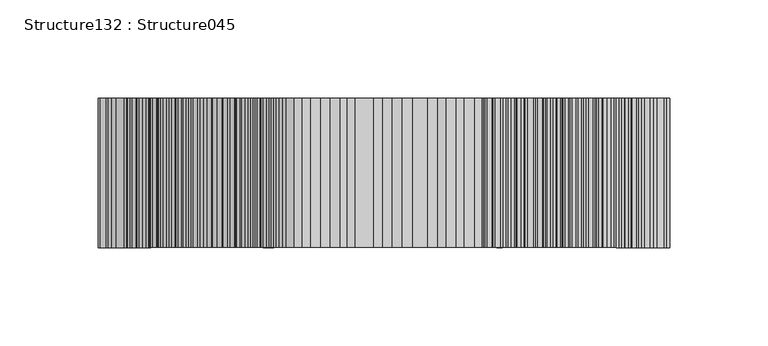
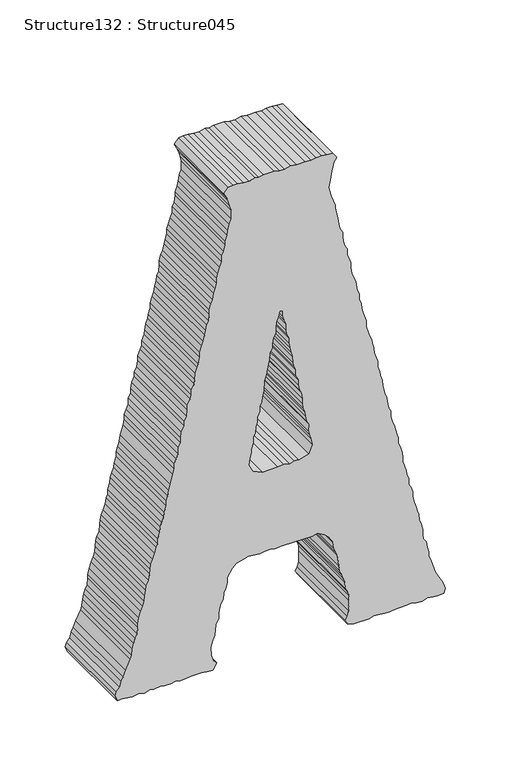
"""IFC4 building model written with IfcOpenShell, lengths in millimetres: proxy geometry, Structure132 : Structure045."""

from ifc_helpers import new_model, si_unit, frame, origin, place, context, project, spatial, polyline, outline, extrude, source, transform, mapped, element, save


def structure132_structure045_523e0b6c(model_context):
    return source(origin(), model_context, "Body", "SweptSolid", [
        extrude(outline(polyline([(3818.8310229, -44517.1979045), (3814.7296538, -44517.1979045), (3811.2043377, -44518.372475), (3805.9476534, -44520.7151975), (3801.8462843, -44520.7151975), (3795.960595, -44521.297669), (3791.8865042, -44523.6387869), (3787.7867397, -44523.6387869), (3783.0868532, -44525.9911371), (3777.8285642, -44526.5655855), (3773.11905, -44526.5655855), (3769.6274306, -44528.9147265), (3763.759392, -44528.9147265), (3759.6596275, -44530.6637454), (3755.559863, -44532.430415), (3750.8583719, -44532.430415), (3746.1745313, -44533.598567), (3737.400554, -44535.9509172), (3732.1149867, -44537.1158601), (3727.4311462, -44538.280803), (3723.3313817, -44539.4585827), (3718.6571688, -44539.4585827), (3713.3555556, -44541.2156246), (3709.2718371, -44541.7997006), (3704.5879966, -44543.5679748), (3701.0723082, -44544.7248946), (3695.786741, -44545.3169937), (3690.512406, -44547.0756402), (3685.8285655, -44547.0756402), (3682.8857208, -44548.2502107), (3677.6274319, -44549.4183628), (3672.9435914, -44551.1850323), (3668.8261762, -44552.9340512), (3664.1423357, -44553.5165226), (3660.0682449, -44554.1086217), (3654.1841602, -44554.6926977), (3650.1004418, -44557.0354203), (3645.9830266, -44557.6162871), (3641.2991861, -44558.2099908), (3636.0408972, -44558.8004853), (3631.915459, -44559.9590097), (3627.8397636, -44561.7256792), (3622.555801, -44563.4843258), (3617.2718384, -44564.6508732), (3613.772196, -44564.6508732), (3607.8961343, -44565.2349493), (3604.3964919, -44567.0016188), (3600.2967274, -44568.1697709), (3595.5872132, -44569.3443414), (3589.7544759, -44569.9284174), (3586.2115092, -44571.0933603), (3577.4535778, -44575.1931248), (3572.1423369, -44577.545475), (3568.6426945, -44579.3041215), (3563.366755, -44580.4690644), (3560.441561, -44583.403886), (3556.3417965, -44584.5784565), (3551.6675836, -44582.8117869), (3551.6675836, -44578.1359694), (3551.0658569, -44573.4441059), (3550.4833855, -44569.3443414), (3551.6675836, -44564.0684018), (3550.4833855, -44558.8004853), (3551.6675836, -44554.1086217), (3551.0658569, -44550.5929333), (3551.6675836, -44544.7248946), (3551.0658569, -44541.2156246), (3551.0658569, -44535.3572136), (3551.6675836, -44531.2574491), (3551.0658569, -44527.1464524), (3551.0658569, -44522.4642164), (3551.6675836, -44517.7803759), (3551.6675836, -44508.4046719), (3551.0658569, -44503.7128083), (3550.4833855, -44498.4448918), (3556.3417965, -44494.9275987), (3559.2669905, -44497.8624203), (3565.1254015, -44499.6210668), (3572.7440636, -44500.1971199), (3578.6104977, -44498.4448918), (3582.7102621, -44496.6782222), (3587.3860796, -44496.0957508), (3592.0955938, -44495.5213024), (3596.7698067, -44493.1689522), (3601.4536473, -44493.1689522), (3604.9709403, -44492.5784577), (3610.2292293, -44491.4119102), (3613.772196, -44489.0627693), (3619.6145609, -44488.4867163), (3622.555801, -44486.7296743), (3627.8397636, -44485.5518946), (3633.0980525, -44485.5518946), (3639.5405396, -44480.8696587), (3643.0578326, -44477.3443426), (3644.8245022, -44470.3177795), (3645.9830266, -44466.8004865), (3645.4262289, -44460.9420755), (3644.8245022, -44456.8407064), (3645.4262289, -44452.1504474), (3645.9830266, -44447.4650023), (3644.8245022, -44443.3748655), (3645.4262289, -44438.0892983), (3645.4262289, -44425.7900048), (3644.8245022, -44419.9299892), (3644.8245022, -44410.5542851), (3645.9830266, -44405.8704446), (3642.4833842, -44399.4199345), (3638.9580681, -44395.32017), (3633.0980525, -44392.3965806), (3627.2396415, -44391.2107779), (3622.555801, -44389.4601544), (3619.6145609, -44388.2871885), (3609.0723094, -44387.1190364), (3604.3964919, -44385.952489), (3600.2967274, -44384.7779185), (3596.1953583, -44383.0176674), (3592.0955938, -44381.8430969), (3586.2115092, -44381.2590208), (3582.7102621, -44379.5019789), (3578.6104977, -44378.3274084), (3573.9266571, -44378.3274084), (3563.9412034, -44378.3274084), (3559.2669905, -44379.5019789), (3555.7416744, -44381.2590208), (3551.6675836, -44378.9195075), (3550.4833855, -44373.6419633), (3550.4833855, -44360.1680993), (3551.6675836, -44356.0667302), (3551.0658569, -44350.7923953), (3550.4833855, -44346.0989271), (3550.4833855, -44342.0071857), (3551.0658569, -44336.139147), (3551.0658569, -44332.0377779), (3551.6675836, -44327.347519), (3551.6675836, -44323.2557775), (3550.4833855, -44318.5735416), (3550.4833855, -44313.2863698), (3551.6675836, -44308.6041339), (3551.0658569, -44303.3378219), (3550.4833855, -44299.8189243), (3551.0658569, -44293.9540948), (3555.1848766, -44292.7859428), (3560.441561, -44294.5349617), (3563.366755, -44295.7207644), (3568.6426945, -44299.2284298), (3572.1423369, -44300.996704), (3576.2693797, -44302.7457229), (3586.2115092, -44305.6693122), (3590.3289243, -44307.4359818), (3594.4286888, -44307.4359818), (3599.1125293, -44308.6041339), (3604.3964919, -44309.7706813), (3608.4705827, -44312.1294499), (3612.5976255, -44312.705503), (3617.2718384, -44312.705503), (3622.555801, -44313.8800735), (3627.2396415, -44315.63872), (3632.5155811, -44316.2211914), (3636.0408972, -44317.3877389), (3640.114988, -44318.5735416), (3645.4262289, -44320.3225605), (3650.6845178, -44321.497131), (3655.3587307, -44321.497131), (3659.4584952, -44322.6717015), (3663.5598643, -44325.0047964), (3668.8261762, -44325.0047964), (3673.5276674, -44326.771466), (3677.0449604, -44327.347519), (3682.8857208, -44329.1141885), (3686.4030139, -44330.288759), (3691.0868544, -44330.288759), (3695.2122926, -44330.8728351), (3699.8881101, -44332.0377779), (3705.7545441, -44334.3901281), (3710.4560353, -44334.3901281), (3714.5301261, -44335.5566756), (3718.0554422, -44336.7312461), (3723.3313817, -44337.9058166), (3727.4311462, -44339.6564401), (3732.7167134, -44340.8326152), (3737.9750024, -44340.8326152), (3740.9162424, -44342.5816341), (3745.6000829, -44343.7562046), (3751.4424479, -44344.3499082), (3756.1423345, -44346.0989271), (3759.6596275, -44347.2734976), (3764.3611187, -44347.8575736), (3769.0176809, -44348.4496727), (3774.3032481, -44350.1986916), (3777.8285642, -44350.7923953), (3783.0868532, -44352.5510418), (3788.3611881, -44352.5510418), (3791.8865042, -44353.7159847), (3797.1463977, -44355.4746312), (3801.8462843, -44356.0667302), (3806.5317294, -44357.2332777), (3810.0474179, -44357.8173538), (3815.3313805, -44360.1680993), (3820.015221, -44361.3330422), (3824.1149855, -44362.5076127), (3829.374879, -44362.5076127), (3837.6000817, -44365.4344113), (3842.8583706, -44366.6089818), (3846.9757858, -44367.2010808), (3851.6612309, -44368.9517043), (3856.9179152, -44368.9517043), (3861.0192843, -44370.7087463), (3866.3032469, -44371.3024499), (3869.8189354, -44371.8833168), (3873.9203044, -44373.6419633), (3878.5784713, -44375.4022144), (3883.8881076, -44376.5687619), (3888.5623205, -44376.5687619), (3892.6636896, -44377.7433324), (3897.3475301, -44379.5019789), (3902.6314927, -44379.5019789), (3906.1487857, -44381.8430969), (3910.8310217, -44383.0176674), (3916.0909152, -44383.5937204), (3919.6066036, -44383.5937204), (3924.2888396, -44385.952489), (3928.9919353, -44387.1190364), (3934.2758979, -44387.7031125), (3938.9517154, -44388.877683), (3944.235678, -44390.0538581), (3947.1496398, -44390.0538581), (3956.5349715, -44393.5711511), (3961.794865, -44394.7264664), (3965.8930249, -44395.9042461), (3974.7055128, -44394.1536226), (3979.9621971, -44392.9774475), (3983.4794902, -44392.3965806), (3987.5792547, -44391.2107779), (3991.6806238, -44388.877683), (3996.390138, -44392.3965806), (3996.9645864, -44397.6709156), (3997.5486624, -44401.7722847), (3997.5486624, -44407.0385967), (3996.390138, -44411.1383611), (3996.9645864, -44416.4223237), (3996.9645864, -44424.0393813), (3997.5486624, -44429.2976702), (3996.390138, -44434.5816328), (3996.390138, -44439.275101), (3997.5486624, -44443.9477093), (3997.5486624, -44453.3234133), (3996.9645864, -44457.4344101), (3997.5486624, -44460.9420755), (3996.390138, -44466.2196197), (3996.390138, -44470.9018556), (3997.5486624, -44476.1761906), (3997.5486624, -44480.2855827), (3996.9645864, -44484.3869518), (3992.2614906, -44488.4867163), (3987.5792547, -44486.1359707), (3984.0635662, -44484.3869518), (3979.3781211, -44483.2123813), (3974.7055128, -44482.0362062), (3966.5043792, -44482.0362062), (3962.3757319, -44483.7932481), (3957.1190475, -44484.9614002), (3952.435207, -44485.5518946), (3947.7337158, -44487.3105412), (3944.235678, -44487.3105412), (3938.3499888, -44488.4867163), (3934.8503464, -44490.2453628), (3929.5904528, -44490.2453628), (3924.8905662, -44492.0040093), (3919.6066036, -44493.7530282), (3915.5068392, -44494.9275987), (3910.8310217, -44494.9275987), (3906.1487857, -44496.0957508), (3902.6314927, -44497.2703213), (3896.763454, -44498.4448918), (3893.822214, -44500.1971199), (3888.5623205, -44501.3716904), (3884.4609514, -44501.3716904), (3878.5784713, -44501.9637894), (3875.0772243, -44503.7128083), (3870.4030114, -44504.2952797), (3866.3032469, -44505.4810825), (3861.0192843, -44506.6460253), (3856.9179152, -44507.8141774), (3851.6612309, -44509.580847), (3846.9757858, -44509.580847), (3841.6741725, -44511.3298659), (3838.1761347, -44511.9123373), (3833.4730389, -44513.6790068), (3828.2163546, -44514.2630829), (3824.1149855, -44514.8471589), (3818.8310229, -44517.1979045)]), holes=[polyline([(3720.4158154, -44454.5092161), (3723.9154578, -44462.700722), (3730.9323932, -44466.2196197), (3736.7988273, -44465.0514676), (3741.5003184, -44463.8768971), (3744.9999608, -44463.8768971), (3750.3015741, -44462.1278782), (3755.559863, -44462.1278782), (3759.0595054, -44460.359604), (3764.3611187, -44459.775528), (3768.4432325, -44458.6009575), (3773.11905, -44458.6009575), (3777.8285642, -44456.2598396), (3783.0868532, -44456.2598396), (3786.0280932, -44454.5092161), (3790.7039107, -44453.917117), (3795.4037973, -44452.7425465), (3804.7730829, -44452.1504474), (3810.0474179, -44450.3998239), (3814.7296538, -44449.8157479), (3818.8310229, -44448.6411774), (3822.932392, -44448.0490784), (3828.790803, -44447.4650023), (3833.4730389, -44445.125489), (3836.9919366, -44445.125489), (3842.2758992, -44444.5317853), (3845.8012153, -44442.1986904), (3851.0595042, -44442.1986904), (3855.7353217, -44441.6081959), (3860.4432313, -44439.8479448), (3865.1190488, -44438.6813973), (3864.5446004, -44436.9147278), (3860.4432313, -44436.9147278), (3856.3161885, -44435.7578079), (3851.6612309, -44433.9911384), (3846.3772683, -44433.9911384), (3842.2758992, -44433.4070623), (3837.6000817, -44431.0643398), (3832.8921721, -44431.0643398), (3828.790803, -44430.4722407), (3824.1149855, -44429.2976702), (3819.4150989, -44428.1407504), (3813.5743386, -44427.5486513), (3810.0474179, -44426.9645753), (3805.9476534, -44425.1963011), (3800.6717138, -44425.1963011), (3795.4037973, -44422.8551832), (3790.7039107, -44422.8551832), (3786.0280932, -44421.6806127), (3782.5027771, -44419.9299892), (3777.2444882, -44419.3459131), (3772.5606477, -44419.3459131), (3767.8607611, -44418.7554187), (3763.759392, -44417.0047952), (3759.6596275, -44416.4223237), (3754.9854146, -44415.8302247), (3750.8583719, -44413.4875021), (3744.9999608, -44414.0619505), (3740.9162424, -44412.9066353), (3736.7988273, -44411.7288556), (3730.9323932, -44410.5542851), (3723.3313817, -44413.4875021), (3720.4158154, -44422.2727117), (3720.9726131, -44426.3740808), (3719.8140887, -44430.4722407), (3720.9726131, -44435.7578079), (3720.4158154, -44441.0241199), (3720.4158154, -44454.5092161)])]), frame((0.0, 247945.1599557, 0.0), z_axis=(0.0, 1.0, 0.0), x_axis=(0.0, 0.0, 1.0)), (0.0, 0.0, 1.0), 76.2),
    ])


if __name__ == "__main__":
    model = new_model("IFC4")
    model_context = context("Model", 3, world=origin())
    ifc_project = project(units=[si_unit("LENGTHUNIT", "METRE", prefix="MILLI")], contexts=[model_context])
    site = spatial("IfcSite", under=ifc_project)
    building = spatial("IfcBuilding", under=site)
    placement = place(None, origin())
    structure132_structure045_shape = structure132_structure045_523e0b6c(model_context)
    element("IfcBuildingElementProxy", 1, Name="Structure132 : Structure045", ObjectType="Structure132 : Structure045", at=placement, inside=building, context=model_context, shape_type="MappedRepresentation", body=[
        mapped(structure132_structure045_shape, transform((0.0, 0.0, 0.0), x_axis=(1.0, 0.0, 0.0), y_axis=(0.0, 1.0, 0.0), z_axis=(0.0, 0.0, 1.0))),
    ])
    save(model, "model.ifc")

# Revit data of these elements
# Type "Structure132 : Structure045"
#   NameOverride = "Structure045"
# Element 1 (IfcBuildingElementProxy, "Structure132 : Structure045")
#   Materials on its faces: "BRUSHED ALUM. LETTERING"
# Materials
#   "BRUSHED ALUM. LETTERING": class "Unassigned", colour RGB 169 181 186, transparency 0, Cost = 0
